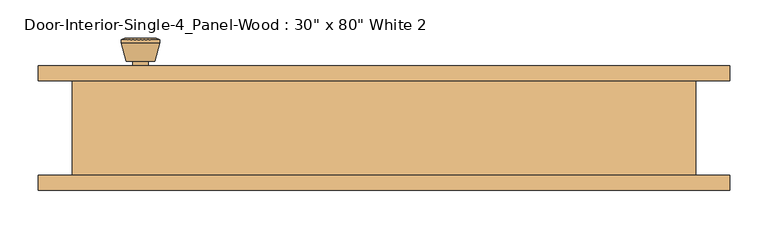
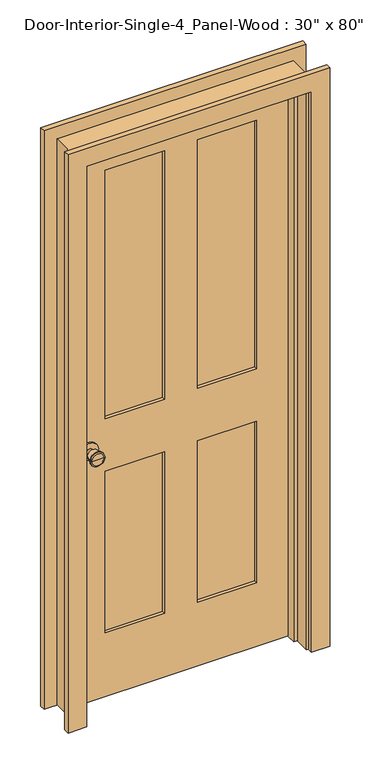
"""IFC4 building model written with IfcOpenShell, lengths in millimetres: door geometry."""

from ifc_helpers import new_model, si_unit, point, frame, frame_2d, origin, place, context, project, spatial, polyline, circle_curve, trimmed, segment, composite_curve, outline, extrude, faceted_brep, source, transform, mapped, element, save
from ifc_brep_helpers import plane_surface, cylinder_surface, revolved_surface, advanced_brep


def door_bbafd44c(model_context):
    return source(origin(), model_context, "Body", "SolidModel", [
        advanced_brep(
        [(-317.5, 17.8125, 914.4), (-307.5, 17.8125, 914.4), (-327.5, 17.8125, 914.4), (-297.0241324, -31.1875, 914.4), (-317.5, -31.1875, 914.4), (-337.9758676, -31.1875, 914.4), (-292.5, -29.3596319, 914.4), (-342.5, -29.3596319, 914.4), (-292.5, -25.8959537, 914.4), (-342.5, -25.8959537, 914.4), (-298.863764, -1.1875, 914.4), (-336.136236, -1.1875, 914.4), (-307.5, -1.1875, 914.4), (-327.5, -1.1875, 914.4)],
        [
            (0, 1),
            (1, 2, circle_curve(frame((-317.5, 17.8125, 914.4), z_axis=(0.0, 1.0, 0.0), x_axis=(-1.0, 0.0, 0.0)), 10.0)),
            (2, 0),
            (2, 1, circle_curve(frame((-317.5, 17.8125, 914.4), z_axis=(0.0, 1.0, 0.0), x_axis=(-1.0, 0.0, 0.0)), 10.0)),
            (3, 4),
            (4, 5),
            (5, 3, circle_curve(frame((-317.5, -31.1875, 914.4), z_axis=(0.0, -1.0, 0.0), x_axis=(-1.0, 0.0, 0.0)), 20.4758676)),
            (3, 5, circle_curve(frame((-317.5, -31.1875, 914.4), z_axis=(0.0, -1.0, 0.0), x_axis=(-1.0, 0.0, 0.0)), 20.4758676)),
            (6, 3),
            (5, 7),
            (7, 6, circle_curve(frame((-317.5, -29.3596319, 914.4), z_axis=(0.0, -1.0, 0.0), x_axis=(-1.0, 0.0, 0.0)), 25.0)),
            (6, 7, circle_curve(frame((-317.5, -29.3596319, 914.4), z_axis=(0.0, -1.0, 0.0), x_axis=(-1.0, 0.0, 0.0)), 25.0)),
            (8, 6),
            (7, 9),
            (9, 8, circle_curve(frame((-317.5, -25.8959537, 914.4), z_axis=(0.0, -1.0, 0.0), x_axis=(-1.0, 0.0, 0.0)), 25.0)),
            (8, 9, circle_curve(frame((-317.5, -25.8959537, 914.4), z_axis=(0.0, -1.0, 0.0), x_axis=(-1.0, 0.0, 0.0)), 25.0)),
            (10, 8),
            (9, 11),
            (11, 10, circle_curve(frame((-317.5, -1.1875, 914.4), z_axis=(0.0, -1.0, 0.0), x_axis=(-1.0, 0.0, 0.0)), 18.636236)),
            (10, 11, circle_curve(frame((-317.5, -1.1875, 914.4), z_axis=(0.0, -1.0, 0.0), x_axis=(-1.0, 0.0, 0.0)), 18.636236)),
            (12, 10),
            (11, 13),
            (13, 12, circle_curve(frame((-317.5, -1.1875, 914.4), z_axis=(0.0, -1.0, 0.0), x_axis=(-1.0, 0.0, 0.0)), 10.0)),
            (12, 13, circle_curve(frame((-317.5, -1.1875, 914.4), z_axis=(0.0, -1.0, 0.0), x_axis=(-1.0, 0.0, 0.0)), 10.0)),
            (1, 12),
            (13, 2),
        ],
        [
            plane_surface(frame((-317.5, 17.8125, 914.4), z_axis=(0.0, 1.0, 0.0), x_axis=(-1.0, 0.0, 0.0))),
            plane_surface(frame((-317.5, -31.1875, 914.4), z_axis=(0.0, -1.0, 0.0), x_axis=(-1.0, 0.0, 0.0))),
            revolved_surface(polyline([(-337.9758676, -31.1875, 914.4), (-342.5, -29.3596319, 914.4)]), (-317.5, 17.8125, 914.4), (0.0, 1.0, 0.0)),
            cylinder_surface(frame((-317.5, 17.8125, 914.4), z_axis=(0.0, 1.0, 0.0), x_axis=(-1.0, 0.0, 0.0)), 25.0),
            revolved_surface(polyline([(-342.5, -25.8959537, 914.4), (-336.136236, -1.1875, 914.4)]), (-317.5, 17.8125, 914.4), (0.0, 1.0, 0.0)),
            plane_surface(frame((-317.5, -1.1875, 914.4), z_axis=(0.0, 1.0, 0.0), x_axis=(-1.0, 0.0, 0.0))),
            cylinder_surface(frame((-317.5, 17.8125, 914.4), z_axis=(0.0, 1.0, 0.0), x_axis=(-1.0, 0.0, 0.0)), 10.0),
        ],
        [
            (0, [[1, 2, 3]]),
            (0, [[-3, 4, -1]]),
            (1, [[5, 6, 7]]),
            (1, [[-6, -5, 8]]),
            (2, [[9, -7, 10, 11]]),
            (2, [[-10, -8, -9, 12]]),
            (3, [[13, -11, 14, 15]]),
            (3, [[-14, -12, -13, 16]]),
            (4, [[17, -15, 18, 19]]),
            (4, [[-18, -16, -17, 20]]),
            (5, [[21, -19, 22, 23]]),
            (5, [[-22, -20, -21, 24]]),
            (6, [[25, -23, 26, -2]]),
            (6, [[-26, -24, -25, -4]]),
        ],
    ),
        extrude(outline(composite_curve([segment(trimmed(circle_curve(frame_2d((914.4, -317.5)), 30.0), [point((914.4, -347.5))], [point((914.4, -287.5))], False, "CARTESIAN"), True, "CONTINUOUS"), segment(trimmed(circle_curve(frame_2d((914.4, -317.5)), 30.0), [point((914.4, -287.5))], [point((914.4, -347.5))], False, "CARTESIAN"), True, "CONTINUOUS")], self_intersect=False)), frame((0.0, 17.8125, 0.0), z_axis=(0.0, 1.0, 0.0), x_axis=(0.0, 0.0, 1.0)), (0.0, 0.0, 1.0), 6.0),
        advanced_brep(
        [(-317.5, 64.7375, 914.4), (-327.5, 64.7375, 914.4), (-307.5, 64.7375, 914.4), (-297.0241324, 113.7375, 914.4), (-337.9758676, 113.7375, 914.4), (-317.5, 113.7375, 914.4), (-292.5, 111.9096319, 914.4), (-342.5, 111.9096319, 914.4), (-292.5, 108.4459537, 914.4), (-342.5, 108.4459537, 914.4), (-298.863764, 83.7375, 914.4), (-336.136236, 83.7375, 914.4), (-307.5, 83.7375, 914.4), (-327.5, 83.7375, 914.4)],
        [
            (0, 1),
            (1, 2, circle_curve(frame((-317.5, 64.7375, 914.4), z_axis=(0.0, -1.0, 0.0), x_axis=(-1.0, 0.0, 0.0)), 10.0)),
            (2, 0),
            (2, 1, circle_curve(frame((-317.5, 64.7375, 914.4), z_axis=(0.0, -1.0, 0.0), x_axis=(-1.0, 0.0, 0.0)), 10.0)),
            (3, 4, circle_curve(frame((-317.5, 113.7375, 914.4), z_axis=(0.0, 1.0, 0.0), x_axis=(-1.0, 0.0, 0.0)), 20.4758676)),
            (4, 5),
            (5, 3),
            (4, 3, circle_curve(frame((-317.5, 113.7375, 914.4), z_axis=(0.0, 1.0, 0.0), x_axis=(-1.0, 0.0, 0.0)), 20.4758676)),
            (6, 7, circle_curve(frame((-317.5, 111.9096319, 914.4), z_axis=(0.0, 1.0, 0.0), x_axis=(-1.0, 0.0, 0.0)), 25.0)),
            (7, 4),
            (3, 6),
            (7, 6, circle_curve(frame((-317.5, 111.9096319, 914.4), z_axis=(0.0, 1.0, 0.0), x_axis=(-1.0, 0.0, 0.0)), 25.0)),
            (8, 9, circle_curve(frame((-317.5, 108.4459537, 914.4), z_axis=(0.0, 1.0, 0.0), x_axis=(-1.0, 0.0, 0.0)), 25.0)),
            (9, 7),
            (6, 8),
            (9, 8, circle_curve(frame((-317.5, 108.4459537, 914.4), z_axis=(0.0, 1.0, 0.0), x_axis=(-1.0, 0.0, 0.0)), 25.0)),
            (10, 11, circle_curve(frame((-317.5, 83.7375, 914.4), z_axis=(0.0, 1.0, 0.0), x_axis=(-1.0, 0.0, 0.0)), 18.636236)),
            (11, 9),
            (8, 10),
            (11, 10, circle_curve(frame((-317.5, 83.7375, 914.4), z_axis=(0.0, 1.0, 0.0), x_axis=(-1.0, 0.0, 0.0)), 18.636236)),
            (12, 13, circle_curve(frame((-317.5, 83.7375, 914.4), z_axis=(0.0, 1.0, 0.0), x_axis=(-1.0, 0.0, 0.0)), 10.0)),
            (13, 11),
            (10, 12),
            (13, 12, circle_curve(frame((-317.5, 83.7375, 914.4), z_axis=(0.0, 1.0, 0.0), x_axis=(-1.0, 0.0, 0.0)), 10.0)),
            (1, 13),
            (12, 2),
        ],
        [
            plane_surface(frame((-317.5, 64.7375, 914.4), z_axis=(0.0, -1.0, 0.0), x_axis=(-1.0, 0.0, 0.0))),
            plane_surface(frame((-317.5, 113.7375, 914.4), z_axis=(0.0, 1.0, 0.0), x_axis=(-1.0, 0.0, 0.0))),
            revolved_surface(polyline([(-337.9758676, 113.7375, 914.4), (-342.5, 111.9096319, 914.4)]), (-317.5, 64.7375, 914.4), (0.0, -1.0, 0.0)),
            cylinder_surface(frame((-317.5, 64.7375, 914.4), z_axis=(0.0, -1.0, 0.0), x_axis=(-1.0, 0.0, 0.0)), 25.0),
            revolved_surface(polyline([(-342.5, 108.4459537, 914.4), (-336.136236, 83.7375, 914.4)]), (-317.5, 64.7375, 914.4), (0.0, -1.0, 0.0)),
            plane_surface(frame((-317.5, 83.7375, 914.4), z_axis=(0.0, -1.0, 0.0), x_axis=(-1.0, 0.0, 0.0))),
            cylinder_surface(frame((-317.5, 64.7375, 914.4), z_axis=(0.0, -1.0, 0.0), x_axis=(-1.0, 0.0, 0.0)), 10.0),
        ],
        [
            (0, [[1, 2, 3]]),
            (0, [[-3, 4, -1]]),
            (1, [[5, 6, 7]]),
            (1, [[8, -7, -6]]),
            (2, [[9, 10, -5, 11]]),
            (2, [[12, -11, -8, -10]]),
            (3, [[13, 14, -9, 15]]),
            (3, [[16, -15, -12, -14]]),
            (4, [[17, 18, -13, 19]]),
            (4, [[20, -19, -16, -18]]),
            (5, [[21, 22, -17, 23]]),
            (5, [[24, -23, -20, -22]]),
            (6, [[-2, 25, -21, 26]]),
            (6, [[-4, -26, -24, -25]]),
        ],
    ),
        extrude(outline(composite_curve([segment(trimmed(circle_curve(frame_2d((914.4, -317.5)), 30.0), [point((914.4, -347.5))], [point((914.4, -287.5))], False, "CARTESIAN"), True, "CONTINUOUS"), segment(trimmed(circle_curve(frame_2d((914.4, -317.5)), 30.0), [point((914.4, -287.5))], [point((914.4, -347.5))], False, "CARTESIAN"), True, "CONTINUOUS")], self_intersect=False)), frame((0.0, 58.7375, 0.0), z_axis=(0.0, 1.0, 0.0), x_axis=(0.0, 0.0, 1.0)), (0.0, 0.0, 1.0), 6.0),
        extrude(outline(polyline([(260.35, 35.4541667), (57.15, 35.4541667), (57.15, 47.0958333), (260.35, 47.0958333), (260.35, 35.4541667)])), frame((0.0, 0.0, 1009.65), z_axis=(0.0, 0.0, 1.0), x_axis=(1.0, 0.0, 0.0)), (0.0, 0.0, 1.0), 903.2875),
        extrude(outline(polyline([(-57.15, 35.4541667), (-260.35, 35.4541667), (-260.35, 47.0958333), (-57.15, 47.0958333), (-57.15, 35.4541667)])), frame((0.0, 0.0, 1009.65), z_axis=(0.0, 0.0, 1.0), x_axis=(1.0, 0.0, 0.0)), (0.0, 0.0, 1.0), 903.2875),
        extrude(outline(polyline([(260.35, 35.4541667), (57.15, 35.4541667), (57.15, 47.0958333), (260.35, 47.0958333), (260.35, 35.4541667)])), frame((0.0, 0.0, 231.775), z_axis=(0.0, 0.0, 1.0), x_axis=(1.0, 0.0, 0.0)), (0.0, 0.0, 1.0), 587.375),
        extrude(outline(polyline([(-57.15, 35.4541667), (-260.35, 35.4541667), (-260.35, 47.0958333), (-57.15, 47.0958333), (-57.15, 35.4541667)])), frame((0.0, 0.0, 231.775), z_axis=(0.0, 0.0, 1.0), x_axis=(1.0, 0.0, 0.0)), (0.0, 0.0, 1.0), 587.375),
        extrude(outline(polyline([(2032.0, -381.0), (0.0, -381.0), (0.0, 381.0), (2032.0, 381.0), (2032.0, -381.0)]), holes=[polyline([(1912.9375, 57.15), (1912.9375, 260.35), (1009.65, 260.35), (1009.65, 57.15), (1912.9375, 57.15)]), polyline([(1009.65, -57.15), (1009.65, -260.35), (1912.9375, -260.35), (1912.9375, -57.15), (1009.65, -57.15)]), polyline([(819.15, 57.15), (819.15, 260.35), (231.775, 260.35), (231.775, 57.15), (819.15, 57.15)]), polyline([(231.775, -57.15), (231.775, -260.35), (819.15, -260.35), (819.15, -57.15), (231.775, -57.15)])]), frame((0.0, 23.8125, 0.0), z_axis=(0.0, 1.0, 0.0), x_axis=(0.0, 0.0, 1.0)), (0.0, 0.0, 1.0), 34.925),
        faceted_brep([(406.4, 58.7375, 0.0), (406.4, -65.0875, 0.0), (381.0, -65.0875, 0.0), (381.0, -11.1125, 0.0), (368.3, -11.1125, 0.0), (368.3, 23.8125, 0.0), (381.0, 23.8125, 0.0), (381.0, 58.7375, 0.0), (406.4, 58.7375, 2057.4), (406.4, -65.0875, 2057.4), (-406.4, -65.0875, 2057.4), (-406.4, -65.0875, 0.0), (-381.0, -65.0875, 0.0), (-381.0, -65.0875, 2032.0), (381.0, -65.0875, 2032.0), (381.0, -11.1125, 2032.0), (-381.0, -11.1125, 2032.0), (-381.0, -11.1125, 0.0), (-368.3, -11.1125, 0.0), (-368.3, -11.1125, 2019.3), (368.3, -11.1125, 2019.3), (368.3, 23.8125, 2019.3), (-368.3, 23.8125, 2019.3), (-368.3, 23.8125, 0.0), (-381.0, 23.8125, 0.0), (-381.0, 23.8125, 2032.0), (381.0, 23.8125, 2032.0), (381.0, 58.7375, 2032.0), (-381.0, 58.7375, 2032.0), (-381.0, 58.7375, 0.0), (-406.4, 58.7375, 0.0), (-406.4, 58.7375, 2057.4)], [[[0, 1, 2, 3, 4, 5, 6, 7]], [[1, 0, 8, 9]], [[2, 1, 9, 10, 11, 12, 13, 14]], [[3, 2, 14, 15]], [[4, 3, 15, 16, 17, 18, 19, 20]], [[5, 4, 20, 21]], [[6, 5, 21, 22, 23, 24, 25, 26]], [[7, 6, 26, 27]], [[0, 7, 27, 28, 29, 30, 31, 8]], [[9, 8, 31, 10]], [[15, 14, 13, 16]], [[21, 20, 19, 22]], [[27, 26, 25, 28]], [[30, 29, 24, 23, 18, 17, 12, 11]], [[10, 31, 30, 11]], [[16, 13, 12, 17]], [[22, 19, 18, 23]], [[28, 25, 24, 29]]]),
        extrude(outline(polyline([(0.0, 387.35), (0.0, 450.85), (2101.85, 450.85), (2101.85, -450.85), (0.0, -450.85), (0.0, -387.35), (2038.35, -387.35), (2038.35, 387.35), (0.0, 387.35)])), frame((0.0, -84.1375, 0.0), z_axis=(0.0, 1.0, 0.0), x_axis=(0.0, 0.0, 1.0)), (0.0, 0.0, 1.0), 19.05),
        extrude(outline(polyline([(0.0, 387.35), (0.0, 450.85), (2101.85, 450.85), (2101.85, -450.85), (0.0, -450.85), (0.0, -387.35), (2038.35, -387.35), (2038.35, 387.35), (0.0, 387.35)])), frame((0.0, 58.7375, 0.0), z_axis=(0.0, 1.0, 0.0), x_axis=(0.0, 0.0, 1.0)), (0.0, 0.0, 1.0), 19.05),
    ])


if __name__ == "__main__":
    model = new_model("IFC4")
    model_context = context("Model", 3, world=origin())
    ifc_project = project(units=[si_unit("LENGTHUNIT", "METRE", prefix="MILLI")], contexts=[model_context])
    site = spatial("IfcSite", under=ifc_project)
    building = spatial("IfcBuilding", under=site)
    placement = place(None, origin())
    door_shape = door_bbafd44c(model_context)
    element("IfcDoor", 1, ObjectType="Door-Interior-Single-4_Panel-Wood : 30\" x 80\" White 2", at=placement, inside=building, context=model_context, shape_type="MappedRepresentation", body=[
        mapped(door_shape, transform((0.0, 0.0, 0.0), x_axis=(1.0, 0.0, 0.0), y_axis=(0.0, 1.0, 0.0), z_axis=(0.0, 0.0, 1.0))),
    ])
    save(model, "model.ifc")

# Revit data of these elements
# Type "Door-Interior-Single-4_Panel-Wood : 30\" x 80\" White 2"
#   Type Mark = "71"
#   COBie.Type.CreatedBy = "doug.wood@us.ibm.com"
#   COBie.Type.CreatedOn = "2016-04-14T02:07:24"
#   COBie.Type.Name = "Doors_Door-Interior-Single-4_Panel-Wood_30\" x 80\" White 2_71"
#   COBie.Type.Category = "23-30 10 00 : Doors"
#   COBie.Type.Description = "Door-Interior-Single-4_Panel-Wood_30\" x 80\" White 2"
#   COBie.Type.Manufacturer = ""
#   COBie.Type.ModelNumber = ""
#   Assembly Code = "C1020300"
#   Analytic Construction = "Wooden"
#   COBie.Type.ReplacementCost = 0
#   Top Rail = 0' - 4 11/16"
#   Thickness = 0' - 1 3/8"
#   Thermal Resistance (R) = 0.455703 (m²·K)/W
#   Swing Angle [instance default] = 90.00°
#   Stiles = 0' - 4 3/4"
#   Rough Width = 2' - 8"
#   Rough Height = 6' - 9"
#   Mullion = 0' - 4 1/2"
#   Lock Rail = 0' - 7 1/2"
#   Height = 6' - 8"
#   Width = 2' - 6"
#   Heat Transfer Coefficient (U) = 2.19465 W/(m²·K)
#   Bottom Rail = 0' - 9 1/8"
#   COBie.Type = no
#   Trim Material = Trim - White
#   Panel Material = Door - Panel - White
#   Frame Material = Door - Panel - White
#   Door Handle Material = ARCAT - Metal - Brass, Polished
#   Visual Light Transmittance = 0
#   Solar Heat Gain Coefficient = 0
#   Wall Closure = (empty or 0)
#   Function = (empty or 0)
# Element 1 (IfcDoor, "Door-Interior-Single-4_Panel-Wood : 30\" x 80\" White 2")
#   Materials on its faces: "Door - Panel - White", "ARCAT - Metal - Brass, Polished", "Trim - White"
# Materials
#   "Trim - White": class "Wood", colour RGB 255 255 255, transparency 0, Cost = 0
#   "Door - Panel - White": class "Wood", colour RGB 255 255 255, transparency 0, Cost = 0
#   "ARCAT - Metal - Brass, Polished": class "Unassigned", colour RGB 246 240 166, transparency 0, Keynote = "05050", Model = "Generic", Manufacturer = "Generic", Description = "Steel, Chrome Plated"
